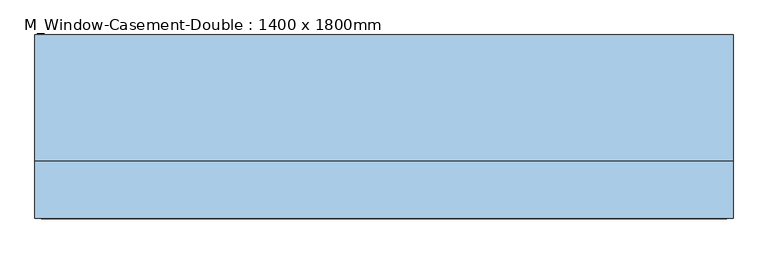
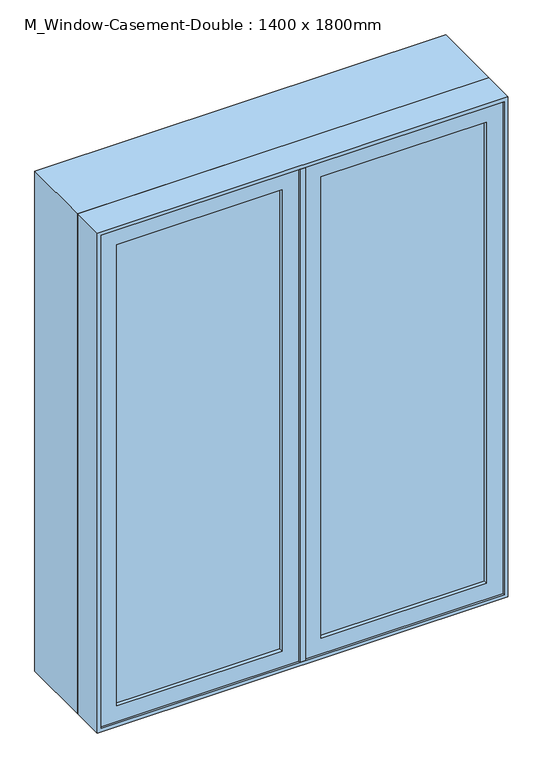
"""IFC4 building model written with IfcOpenShell, lengths in millimetres: window geometry, M_Window-Casement-Double : 1400 x 1800mm."""

from ifc_helpers import new_model, si_unit, frame, origin, place, context, project, spatial, polyline, outline, extrude, faceted_brep, source, transform, mapped, element, save


def m_window_casement_double_1400_x_1800mm_42382f28(model_context):
    return source(origin(), model_context, "Body", "SolidModel", [
        faceted_brep([(668.25, -142.75, 2668.25), (-668.25, -142.75, 2668.25), (-668.25, -79.25, 2668.25), (668.25, -79.25, 2668.25), (687.3, -193.55, 2687.3), (-687.3, -193.55, 2687.3), (-687.3, -142.75, 2687.3), (687.3, -142.75, 2687.3), (700.0, -79.25, 2700.0), (-700.0, -79.25, 2700.0), (-700.0, -193.55, 2700.0), (700.0, -193.55, 2700.0), (-668.25, -142.75, 931.75), (-668.25, -79.25, 931.75), (-687.3, -193.55, 912.7), (-687.3, -142.75, 912.7), (-700.0, -79.25, 900.0), (-700.0, -193.55, 900.0), (668.25, -142.75, 931.75), (668.25, -79.25, 931.75), (687.3, -193.55, 912.7), (687.3, -142.75, 912.7), (700.0, -79.25, 900.0), (700.0, -193.55, 900.0)], [[[0, 1, 2, 3]], [[4, 5, 6, 7]], [[8, 9, 10, 11]], [[1, 12, 13, 2]], [[5, 14, 15, 6]], [[9, 16, 17, 10]], [[12, 18, 19, 13]], [[14, 20, 21, 15]], [[16, 22, 23, 17]], [[9, 8, 22, 16], [3, 2, 13, 19]], [[18, 0, 3, 19]], [[7, 6, 15, 21], [1, 0, 18, 12]], [[20, 4, 7, 21]], [[22, 8, 11, 23]], [[11, 10, 17, 23], [5, 4, 20, 14]]]),
        extrude(outline(polyline([(2700.0, -700.0), (900.0, -700.0), (900.0, 700.0), (2700.0, 700.0), (2700.0, -700.0)]), holes=[polyline([(2680.95, 680.95), (919.05, 680.95), (919.05, -680.95), (2680.95, -680.95), (2680.95, 680.95)])]), frame((0.0, -79.25, 0.0), z_axis=(0.0, 1.0, 0.0), x_axis=(0.0, 0.0, 1.0)), (0.0, 0.0, 1.0), 253.75),
        extrude(outline(polyline([(912.7, 9.525), (912.7, 687.3), (2687.3, 687.3), (2687.3, 9.525), (912.7, 9.525)]), holes=[polyline([(969.85, 630.15), (969.85, 66.675), (2630.15, 66.675), (2630.15, 630.15), (969.85, 630.15)])]), frame((0.0, -187.2, 0.0), z_axis=(0.0, 1.0, 0.0), x_axis=(0.0, 0.0, 1.0)), (0.0, 0.0, 1.0), 44.45),
        extrude(outline(polyline([(2687.3, -9.525), (2687.3, -687.3), (912.7, -687.3), (912.7, -9.525), (2687.3, -9.525)]), holes=[polyline([(2630.15, -630.15), (2630.15, -66.675), (969.85, -66.675), (969.85, -630.15), (2630.15, -630.15)])]), frame((0.0, -187.2, 0.0), z_axis=(0.0, 1.0, 0.0), x_axis=(0.0, 0.0, 1.0)), (0.0, 0.0, 1.0), 44.45),
        extrude(outline(polyline([(630.15, -174.5), (66.675, -174.5), (66.675, -168.15), (630.15, -168.15), (630.15, -174.5)])), frame((0.0, 0.0, 969.85), z_axis=(0.0, 0.0, 1.0), x_axis=(1.0, 0.0, 0.0)), (0.0, 0.0, 1.0), 1660.3),
        extrude(outline(polyline([(66.675, -155.45), (630.15, -155.45), (630.15, -161.8), (66.675, -161.8), (66.675, -155.45)])), frame((0.0, 0.0, 969.85), z_axis=(0.0, 0.0, 1.0), x_axis=(1.0, 0.0, 0.0)), (0.0, 0.0, 1.0), 1660.3),
        extrude(outline(polyline([(-66.675, -174.5), (-630.15, -174.5), (-630.15, -168.15), (-66.675, -168.15), (-66.675, -174.5)])), frame((0.0, 0.0, 969.85), z_axis=(0.0, 0.0, 1.0), x_axis=(1.0, 0.0, 0.0)), (0.0, 0.0, 1.0), 1660.3),
        extrude(outline(polyline([(-630.15, -155.45), (-66.675, -155.45), (-66.675, -161.8), (-630.15, -161.8), (-630.15, -155.45)])), frame((0.0, 0.0, 969.85), z_axis=(0.0, 0.0, 1.0), x_axis=(1.0, 0.0, 0.0)), (0.0, 0.0, 1.0), 1660.3),
        faceted_brep([(9.525, -193.55, 2687.3), (9.525, -142.75, 2687.3), (-9.525, -142.75, 2687.3), (-9.525, -193.55, 2687.3), (9.525, -193.55, 912.7), (-9.525, -193.55, 912.7), (-9.525, -142.75, 912.7), (9.525, -142.75, 912.7), (-9.525, -142.75, 2668.25), (-9.525, -142.75, 931.75), (-30.1625, -142.75, 2668.25), (-30.1625, -142.75, 931.75), (-30.1625, -79.25, 2668.25), (-30.1625, -79.25, 931.75), (30.1625, -79.25, 2668.25), (30.1625, -79.25, 931.75), (30.1625, -142.75, 2668.25), (30.1625, -142.75, 931.75), (9.525, -142.75, 2668.25), (9.525, -142.75, 931.75)], [[[0, 1, 2, 3]], [[4, 5, 6, 7]], [[3, 5, 4, 0]], [[2, 8, 9, 6, 5, 3]], [[8, 10, 11, 9]], [[10, 12, 13, 11]], [[12, 14, 15, 13]], [[14, 16, 17, 15]], [[16, 18, 19, 17]], [[0, 4, 7, 19, 18, 1]], [[8, 2, 1, 18]], [[19, 7, 6, 9]], [[9, 11, 13, 15, 17, 19]], [[18, 16, 14, 12, 10, 8]]]),
    ])


if __name__ == "__main__":
    model = new_model("IFC4")
    model_context = context("Model", 3, world=origin())
    ifc_project = project(units=[si_unit("LENGTHUNIT", "METRE", prefix="MILLI")], contexts=[model_context])
    site = spatial("IfcSite", under=ifc_project)
    building = spatial("IfcBuilding", under=site)
    placement = place(None, origin())
    m_window_casement_double_1400_x_1800mm_shape = m_window_casement_double_1400_x_1800mm_42382f28(model_context)
    element("IfcWindow", 1, ObjectType="M_Window-Casement-Double : 1400 x 1800mm", at=placement, inside=building, context=model_context, shape_type="MappedRepresentation", body=[
        mapped(m_window_casement_double_1400_x_1800mm_shape, transform((0.0, 0.0, 0.0), x_axis=(1.0, 0.0, 0.0), y_axis=(0.0, 1.0, 0.0), z_axis=(0.0, 0.0, 1.0))),
    ])
    save(model, "model.ifc")

# Revit data of these elements
# Type "M_Window-Casement-Double : 1400 x 1800mm"
#   Type Mark = "27"
#   Fire Rating = "0.5h"
#   Assembly Code = "B2020100"
#   Analytic Construction = "Double glazing - domestic"
#   Frame Extension [instance default] = 6.35 mm
#   Window Inset [instance default] = 0 mm
#   Wall Thickness [instance default] = 150 mm
#   Interior Wall Closure [instance default] = 54.75 mm
#   Half Width = 700 mm
#   Visual Light Transmittance = 0.81
#   Thermal Resistance (R) = 0.319569 (m²·K)/W
#   Solar Heat Gain Coefficient = 0.76
#   Rough Width = 1415 mm
#   Rough Height = 1815 mm
#   Height = 1800 mm
#   Heat Transfer Coefficient (U) = 3.12929 W/(m²·K)
#   Exterior Wall Closure [instance default] = 31.8 mm
#   Extension Jamb [instance default] = 54.75 mm
#   Default Sill Height = 900 mm
#   Width = 1400 mm
#   Muntin Visibility = yes
#   Interior Trim Visibility [instance default] = yes
#   Exterior Trim Visibility [instance default] = yes
#   Extension Jamb Visibility [instance default] = yes
#   Interior Trim Material = Wood - Stained
#   Muntin Pattern = M_Muntin Pattern_2x2 : M_Muntin Pattern_2x2
#   Interior Trim = M_Trim-Window-Interior-Flat : Picture Frame
#   Interior Frame Material = Wood - Stained
#   Glass Panel Material = Glass
#   Exterior Trim Material = Clad - White
#   Exterior Trim = M_Trim-Window-Exterior-Flat : with Sill
#   Exterior Frame Material = Clad - White
#   Wall Closure = (empty or 0)
# Element 1 (IfcWindow, "M_Window-Casement-Double : 1400 x 1800mm")
#   Wall Thickness = 349 mm
#   Extension Jamb = 253.75 mm
#   Materials on its faces: "Wood - Stained", "Glass", "Clad - White"
# Materials
#   "Wood - Stained": class "Wood", colour RGB 173 132 96, transparency 0, Cost = 0
#   "Glass": class "Glass", colour RGB 245 245 243, transparency 1, Description = "Soda Lime Glass", Cost = 0
#   "Clad - White": class "Wood", colour RGB 245 245 243, transparency 0, Cost = 0
